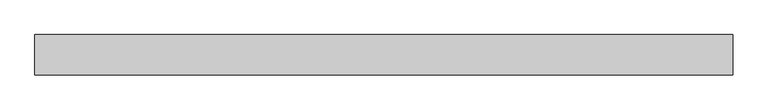
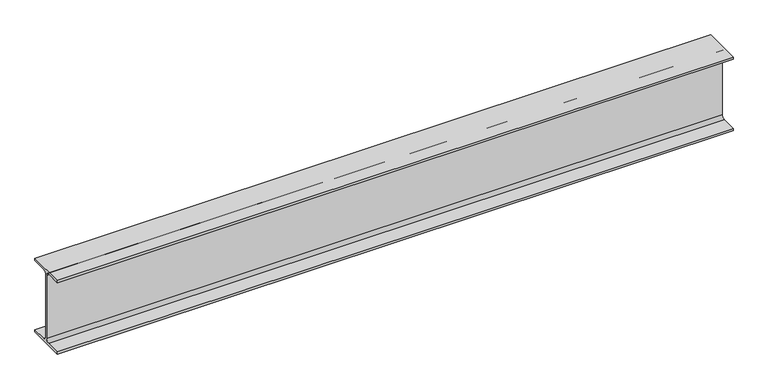
"""IFC4 building model written with IfcOpenShell, lengths in millimetres: beam geometry, Steel Framing_H_KS : H_SB_AR_S02_H-300x150x6.5x9_WG1."""

from ifc_helpers import new_model, si_unit, point, frame, frame_2d, origin, place, context, project, spatial, polyline, circle_curve, trimmed, segment, composite_curve, outline, extrude, source, transform, mapped, element, save


def beam_7b708543(model_context):
    return source(origin(), model_context, "Body", "SweptSolid", [
        extrude(outline(composite_curve([segment(polyline([(75.0, -141.0), (75.0, -150.0), (-75.0, -150.0), (-75.0, -141.0), (-16.25, -141.0)]), True, "CONTINUOUS"), segment(trimmed(circle_curve(frame_2d((-16.25, -128.0)), 13.0), [point((-16.25, -141.0))], [point((-3.25, -128.0))], True, "CARTESIAN"), True, "CONTINUOUS"), segment(polyline([(-3.25, -128.0), (-3.25, 128.0)]), True, "CONTINUOUS"), segment(trimmed(circle_curve(frame_2d((-16.25, 128.0)), 13.0), [point((-3.25, 128.0))], [point((-16.25, 141.0))], True, "CARTESIAN"), True, "CONTINUOUS"), segment(polyline([(-16.25, 141.0), (-75.0, 141.0), (-75.0, 150.0), (75.0, 150.0), (75.0, 141.0), (16.25, 141.0)]), True, "CONTINUOUS"), segment(trimmed(circle_curve(frame_2d((16.25, 128.0)), 13.0), [point((16.25, 141.0))], [point((3.25, 128.0))], True, "CARTESIAN"), True, "CONTINUOUS"), segment(polyline([(3.25, 128.0), (3.25, -128.0)]), True, "CONTINUOUS"), segment(trimmed(circle_curve(frame_2d((16.25, -128.0)), 13.0), [point((3.25, -128.0))], [point((16.25, -141.0))], True, "CARTESIAN"), True, "CONTINUOUS"), segment(polyline([(16.25, -141.0), (75.0, -141.0)]), True, "CONTINUOUS")], self_intersect=False)), frame((-1412.3, 0.0, 0.0), z_axis=(1.0, 0.0, 0.0), x_axis=(0.0, 1.0, 0.0)), (0.0, 0.0, 1.0), 2605.6),
    ])


if __name__ == "__main__":
    model = new_model("IFC4")
    model_context = context("Model", 3, world=origin())
    ifc_project = project(units=[si_unit("LENGTHUNIT", "METRE", prefix="MILLI")], contexts=[model_context])
    site = spatial("IfcSite", under=ifc_project)
    building = spatial("IfcBuilding", under=site)
    placement = place(None, origin())
    beam_shape = beam_7b708543(model_context)
    element("IfcBeam", 1, ObjectType="Steel Framing_H_KS : H_SB_AR_S02_H-300x150x6.5x9_WG1", at=placement, inside=building, context=model_context, shape_type="MappedRepresentation", body=[
        mapped(beam_shape, transform((0.0, 0.0, 0.0), x_axis=(1.0, 0.0, 0.0), y_axis=(0.0, 1.0, 0.0), z_axis=(0.0, 0.0, 1.0))),
    ])
    save(model, "model.ifc")

# Revit data of these elements
# Type "Steel Framing_H_KS : H_SB_AR_S02_H-300x150x6.5x9_WG1"
#   Type Comments = "MAIN"
#   Type Mark = "WG1"
#   H_SectionID = "H-300x150x6.5x9"
#   H_Ratio for Additional Steel Plate = 0.2
#   Width = 15.0 cm
#   Web Thickness = 0.65 cm
#   Web Fillet = 1.3 cm
#   Warping Constant = 107000.0 cm⁶
#   Torsional Moment of Inertia = 9.9539 cm⁴
#   Section Area = 46.78 cm²
#   Plastic Modulus weak axis = 105.0 cm³
#   Plastic Modulus strong axis = 542.0 cm³
#   Perimeter = 1.17 m²/m
#   Nominal Weight = 36.70 kgf/m
#   Moment of Inertia weak axis = 508.00 cm⁴
#   Moment of Inertia strong axis = 7210.00 cm⁴
#   Height = 30.0 cm
#   Flange Thickness = 0.9 cm
#   Elastic Modulus weak axis = 67.7 cm³
#   Elastic Modulus strong axis = 481.0 cm³
#   Centroid Vertical = 15.0 cm
#   Centroid Horizontal = 7.5 cm
#   Bolt Spacing = 8.89 cm
#   Length [instance default] = 1500 mm
#   Structural Material [instance default] = Steel, 45-345
#   Section Name Key = ""
#   Assembly Code = ""
# Element 1 (IfcBeam, "Steel Framing_H_KS : H_SB_AR_S02_H-300x150x6.5x9_WG1")
#   Materials on its faces: "Steel, 45-345"
# Materials
#   "Steel, 45-345": class "Metal", colour RGB 189 187 185, transparency 0, Description = "Steel 345 MPa", Cost = 0
